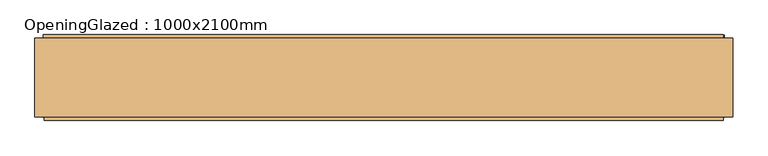
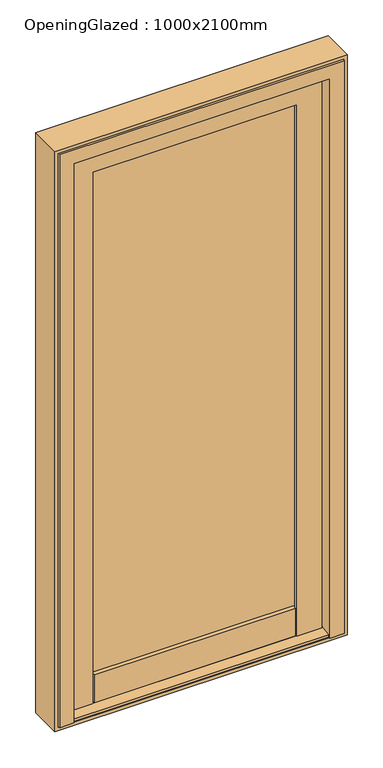
"""IFC4 building model written with IfcOpenShell, lengths in millimetres: door geometry, OpeningGlazed : 1000x2100mm."""

import ifcopenshell
import ifcopenshell.guid

model = None  # the IFC model being written
_history = None  # IfcOwnerHistory: only IFC2X3 demands one
_inside = {}  # id of a spatial element -> (the spatial element, [elements in it])
_under = {}  # id of a project, library or spatial element -> (it, [spatial elements below it])
_declared = {}  # id of a project -> (the project, [libraries it declares])
_typed = {}  # id of a type object -> (the type object, [elements of that type])
_made_of = {}  # id of a material, layer set ... -> (it, [elements and type objects made of it])


def new_model(schema):
    """Start an empty IFC model of exactly this schema.

    Asked for "IFC4X3", IfcOpenShell would pick the latest addendum, in which some entities
    have other attributes; the version numbers below select the first issue.
    IFC2X3 requires an IfcOwnerHistory on every rooted entity: one is made here for all.
    """
    global model, _history
    if schema == "IFC4X3":
        model = ifcopenshell.file(schema_version=(4, 3, 0, 0))
    else:
        model = ifcopenshell.file(schema=schema)
    _inside.clear()
    _under.clear()
    _declared.clear()
    _typed.clear()
    _made_of.clear()
    _history = None
    if model.schema == "IFC2X3":
        org = make("IfcOrganization", Name="unknown")
        user = make(
            "IfcPersonAndOrganization",
            ThePerson=make("IfcPerson", FamilyName="unknown"),
            TheOrganization=org,
        )
        app = make(
            "IfcApplication",
            ApplicationDeveloper=org,
            Version="unknown",
            ApplicationFullName="unknown",
            ApplicationIdentifier="unknown",
        )
        _history = make(
            "IfcOwnerHistory",
            OwningUser=user,
            OwningApplication=app,
            ChangeAction="ADDED",
            CreationDate=0,
        )
    return model


def make(cls, **values):
    """One entity of the class cls with the attributes given. An attribute that is None is left unset."""
    return model.create_entity(
        cls, **{name: value for name, value in values.items() if value is not None}
    )


def rooted(cls, **values):
    """An entity with a GlobalId (a new one), such as an element, a storey or a relation."""
    return make(cls, GlobalId=ifcopenshell.guid.new(), OwnerHistory=_history, **values)


def si_unit(unit_type, name, prefix=None):
    """IfcSIUnit, for example si_unit("LENGTHUNIT", "METRE", prefix="MILLI")."""
    return make("IfcSIUnit", UnitType=unit_type, Prefix=prefix, Name=name)


def assignment(units):
    """IfcUnitAssignment: the units of a project."""
    return None if units is None else make("IfcUnitAssignment", Units=units)


def point(xyz):
    """IfcCartesianPoint."""
    return None if xyz is None else make("IfcCartesianPoint", Coordinates=xyz)


def direction(xyz):
    """IfcDirection."""
    return None if xyz is None else make("IfcDirection", DirectionRatios=xyz)


def frame(location, z_axis=None, x_axis=None):
    """IfcAxis2Placement3D, a coordinate frame: its origin and axes. An axis left out is left unset."""
    return make(
        "IfcAxis2Placement3D",
        Location=point(location),
        Axis=direction(z_axis),
        RefDirection=direction(x_axis),
    )


def origin():
    """The frame at (0, 0, 0) with its axes left unset."""
    return frame((0.0, 0.0, 0.0))


def place(relative_to, where):
    """IfcLocalPlacement: puts the frame where relative to a parent placement (None: the world)."""
    return make(
        "IfcLocalPlacement", PlacementRelTo=relative_to, RelativePlacement=where
    )


def context(
    kind, dimensions, precision=None, world=None, true_north=None, identifier=None
):
    """IfcGeometricRepresentationContext, for example the 3D "Model" context."""
    return make(
        "IfcGeometricRepresentationContext",
        ContextIdentifier=identifier,
        ContextType=kind,
        CoordinateSpaceDimension=dimensions,
        Precision=precision,
        WorldCoordinateSystem=world,
        TrueNorth=true_north,
    )


def project(units=None, contexts=None):
    """IfcProject with its units and contexts."""
    return rooted(
        "IfcProject",
        Name="project",
        RepresentationContexts=contexts,
        UnitsInContext=assignment(units),
    )


def spatial(cls, under=None, at=None, **own):
    """A site, building, storey or space (cls), placed at a placement, below another one or the project."""
    s = rooted(cls, ObjectPlacement=at, **own)
    if under is not None:
        _under.setdefault(under.id(), (under, []))[1].append(s)
    return s


def polyline(points):
    """IfcPolyline through the points."""
    return make("IfcPolyline", Points=[point(p) for p in points])


def outline(outer, holes=None, kind="AREA"):
    """IfcArbitraryClosedProfileDef: a profile drawn as a closed curve; with holes, ...WithVoids."""
    if holes is None:
        return make("IfcArbitraryClosedProfileDef", ProfileType=kind, OuterCurve=outer)
    return make(
        "IfcArbitraryProfileDefWithVoids",
        ProfileType=kind,
        OuterCurve=outer,
        InnerCurves=holes,
    )


def extrude(swept, where, along, depth):
    """IfcExtrudedAreaSolid: the profile swept, set in the frame where, extruded along a direction by depth."""
    return make(
        "IfcExtrudedAreaSolid",
        SweptArea=swept,
        Position=where,
        ExtrudedDirection=direction(along),
        Depth=depth,
    )


def faces_of(points, faces, orient=None, outer=None):
    """IfcFace entities. A face is a list of loops; a loop is a list of indices into points, from 0.

    orient and outer hold one flag for each loop. By default every Orientation is true, the
    first loop of a face is its IfcFaceOuterBound and the others are IfcFaceBound.
    """
    made = []
    for i, loops in enumerate(faces):
        bounds = []
        for j, loop in enumerate(loops):
            is_outer = j == 0 if outer is None else outer[i][j]
            bounds.append(
                make(
                    "IfcFaceOuterBound" if is_outer else "IfcFaceBound",
                    Bound=make("IfcPolyLoop", Polygon=[points[k] for k in loop]),
                    Orientation=True if orient is None else orient[i][j],
                )
            )
        made.append(make("IfcFace", Bounds=bounds))
    return made


def faceted_brep(points, faces, orient=None, outer=None, voids=None):
    """IfcFacetedBrep: a solid bounded by flat faces; with voids (closed shells), ...WithVoids."""
    shared = [point(p) for p in points]
    hull = make("IfcClosedShell", CfsFaces=faces_of(shared, faces, orient, outer))
    if voids is None:
        return make("IfcFacetedBrep", Outer=hull)
    return make(
        "IfcFacetedBrepWithVoids",
        Outer=hull,
        Voids=[
            make(cls, CfsFaces=faces_of(shared, fs, o, b)) for cls, fs, o, b in voids
        ],
    )


def shape(context_of_items, identifier, shape_type, items):
    """IfcShapeRepresentation: the items that make up one representation, for example the "Body"."""
    return make(
        "IfcShapeRepresentation",
        ContextOfItems=context_of_items,
        RepresentationIdentifier=identifier,
        RepresentationType=shape_type,
        Items=items,
    )


def source(mapping_origin, context_of_items, identifier, shape_type, items):
    """IfcRepresentationMap: a shape defined once, which mapped items show again and again."""
    return make(
        "IfcRepresentationMap",
        MappingOrigin=mapping_origin,
        MappedRepresentation=shape(context_of_items, identifier, shape_type, items),
    )


def transform(
    local_origin,
    x_axis=None,
    y_axis=None,
    z_axis=None,
    scale=None,
    scale2=None,
    scale3=None,
    uniform=True,
):
    """IfcCartesianTransformationOperator3D, or its non-uniform kind. x_axis, y_axis, z_axis: its Axis1, 2, 3."""
    if uniform:
        return make(
            "IfcCartesianTransformationOperator3D",
            Axis1=direction(x_axis),
            Axis2=direction(y_axis),
            LocalOrigin=point(local_origin),
            Scale=scale,
            Axis3=direction(z_axis),
        )
    return make(
        "IfcCartesianTransformationOperator3DnonUniform",
        Axis1=direction(x_axis),
        Axis2=direction(y_axis),
        LocalOrigin=point(local_origin),
        Scale=scale,
        Axis3=direction(z_axis),
        Scale2=scale2,
        Scale3=scale3,
    )


def mapped(mapping_source, mapping_target):
    """IfcMappedItem: shows the shape of a source again, moved by a transform."""
    return make(
        "IfcMappedItem", MappingSource=mapping_source, MappingTarget=mapping_target
    )


def made_of(thing, what):
    """Note that an element or type object is made of a material, layer set ...; save() writes the relation."""
    if what is not None:
        _made_of.setdefault(what.id(), (what, []))[1].append(thing)
    return thing


def element(
    cls,
    number,
    at=None,
    inside=None,
    cuts=None,
    type_object=None,
    material=None,
    context=None,
    identifier="Body",
    shape_type=None,
    held_by="IfcProductDefinitionShape",
    body=None,
    shapes=None,
    **own,
):
    """One element of the class cls, such as IfcWall. Its Tag is "e" and its number.

    at: its placement. inside: the storey or other place that contains it. cuts: it is an
    opening in that element (IfcRelVoidsElement). A single representation is given by context,
    identifier, shape_type and body (its items); several are given by shapes. held_by: the class
    of the entity that holds the representations. save() writes the other relations.
    """
    e = rooted(cls, Tag="e%d" % number, ObjectPlacement=at, **own)
    if body is not None:
        shapes = [shape(context, identifier, shape_type, body)]
    if shapes is not None:
        e.Representation = make(held_by, Representations=shapes)
    if inside is not None:
        _inside.setdefault(inside.id(), (inside, []))[1].append(e)
    if cuts is not None:
        rooted(
            "IfcRelVoidsElement", RelatingBuildingElement=cuts, RelatedOpeningElement=e
        )
    if type_object is not None:
        _typed.setdefault(type_object.id(), (type_object, []))[1].append(e)
    return made_of(e, material)


def aggregate(whole, parts):
    """IfcRelAggregates: a whole, such as a stair, and the parts it consists of."""
    return rooted("IfcRelAggregates", RelatingObject=whole, RelatedObjects=parts)


def save(model, path):
    """Write the relations noted so far, then the file.

    IfcRelAggregates (storeys below a building ...), IfcRelContainedInSpatialStructure (elements
    in a storey), IfcRelDefinesByType, IfcRelAssociatesMaterial and IfcRelDeclares: one each for
    every whole, place, type object, material and project.
    """
    for whole, parts in _under.values():
        aggregate(whole, parts)
    for where, things in _inside.values():
        rooted(
            "IfcRelContainedInSpatialStructure",
            RelatedElements=things,
            RelatingStructure=where,
        )
    for kind, things in _typed.values():
        rooted("IfcRelDefinesByType", RelatedObjects=things, RelatingType=kind)
    for what, things in _made_of.values():
        rooted("IfcRelAssociatesMaterial", RelatedObjects=things, RelatingMaterial=what)
    for by, libraries in _declared.values():
        rooted("IfcRelDeclares", RelatingContext=by, RelatedDefinitions=libraries)
    model.write(path)


def openingglazed_1000x2100mm_71b3a25b(model_context):
    return source(origin(), model_context, "Body", "SolidModel", [
        extrude(outline(polyline([(40.9999982, 133.0208766), (48.9999995, 130.8772832), (48.9999995, 112.2614733), (47.8757378, 111.1372136), (48.9999995, 110.0129457), (48.9999995, 21.4372109), (40.9999982, 21.4372109), (40.9999982, 133.0208766)])), frame((-488.0, 0.0, 0.0), z_axis=(1.0, 0.0, 0.0), x_axis=(0.0, 1.0, 0.0)), (0.0, 0.0, 1.0), 976.0),
        extrude(outline(polyline([(-16.0, 18.5055334), (50.0, 14.6999975), (50.0, 12.0), (-65.0000006, 12.0), (-65.0000006, 21.5000005), (-28.9462261, 25.9268477), (-28.000001, 28.5265826), (-16.0, 30.0000015), (-16.0, 18.5055334)])), frame((-488.0, 0.0, 0.0), z_axis=(1.0, 0.0, 0.0), x_axis=(0.0, 1.0, 0.0)), (0.0, 0.0, 1.0), 976.0),
        extrude(outline(polyline([(40.9999982, 108.2792699), (40.9999982, 15.2189343), (-16.0, 18.5055334), (-16.0, 30.0000015), (-31.0000006, 28.1582279), (-31.0000006, 129.0), (2.9999994, 133.0), (2.9999994, 112.9450831), (40.9999982, 108.2792699)])), frame((-344.5316437, 0.0, 0.0), z_axis=(1.0, 0.0, 0.0), x_axis=(0.0, 1.0, 0.0)), (0.0, 0.0, 1.0), 689.0632873),
        extrude(outline(polyline([(358.6999971, 37.9999995), (358.6999971, 33.9999989), (-358.6999971, 33.9999989), (-358.6999971, 37.9999995), (358.6999971, 37.9999995)])), frame((0.0, 0.0, 121.9447729), z_axis=(0.0, 0.0, 1.0), x_axis=(1.0, 0.0, 0.0)), (0.0, 0.0, 1.0), 1836.7552241),
        extrude(outline(polyline([(358.6999971, -15.0000005), (358.6999971, -19.0000005), (-358.6999971, -19.0000005), (-358.6999971, -15.0000005), (358.6999971, -15.0000005)])), frame((0.0, 0.0, 121.9447729), z_axis=(0.0, 0.0, 1.0), x_axis=(1.0, 0.0, 0.0)), (0.0, 0.0, 1.0), 1836.7552241),
        extrude(outline(polyline([(2100.0, 500.0), (2100.0, -500.0), (0.0, -500.0), (0.0, 500.0), (2100.0, 500.0)]), holes=[polyline([(12.0, 488.0), (12.0, -488.0), (2088.0, -488.0), (2088.0, 488.0), (12.0, 488.0)])]), frame((0.0, -68.0, 0.0), z_axis=(0.0, 1.0, 0.0), x_axis=(0.0, 0.0, 1.0)), (0.0, 0.0, 1.0), 113.0),
        faceted_brep([(486.7916962, 41.6999992, 13.2083038), (486.7916962, -73.3, 13.2083038), (437.9999993, -73.3, 13.2083038), (437.9999993, -16.0, 13.2083038), (455.8269997, -16.0, 13.2083038), (462.9116684, 41.6999992, 13.2083038), (-486.7916962, 41.6999992, 13.2083038), (-462.9116684, 41.6999992, 13.2083038), (-455.8269997, -16.0, 13.2083038), (-437.9999993, -16.0, 13.2083038), (-437.9999993, -73.3, 13.2083038), (-486.7916962, -73.3, 13.2083038), (462.9116684, 41.6999992, 2062.9116684), (-462.9116684, 41.6999992, 2062.9116684), (-486.7916962, 41.6999992, 2086.7916962), (486.7916962, 41.6999992, 2086.7916962), (486.7916962, -73.3, 2086.7916962), (-486.7916962, -73.3, 2086.7916962), (-437.9999993, -73.3, 2037.9999993), (437.9999993, -73.3, 2037.9999993), (437.9999993, -16.0, 2037.9999993), (-437.9999993, -16.0, 2037.9999993), (-455.8269997, -16.0, 2055.8269997), (455.8269997, -16.0, 2055.8269997)], [[[0, 1, 2, 3, 4, 5]], [[6, 7, 8, 9, 10, 11]], [[0, 5, 12, 13, 7, 6, 14, 15]], [[1, 0, 15, 16]], [[2, 1, 16, 17, 11, 10, 18, 19]], [[16, 15, 14, 17]], [[17, 14, 6, 11]], [[3, 2, 19, 20]], [[4, 3, 20, 21, 9, 8, 22, 23]], [[5, 4, 23, 12]], [[20, 19, 18, 21]], [[12, 23, 22, 13]], [[21, 18, 10, 9]], [[13, 22, 8, 7]]]),
        faceted_brep([(450.532936, -11.0000001, 13.2083038), (434.0000042, -11.0000001, 13.2083038), (434.0000042, -31.0000006, 13.2083038), (348.9999993, -31.0000006, 13.2083038), (345.0, 2.9999994, 13.2083038), (365.1556953, 2.9999994, 13.2083038), (369.8215082, 40.9999982, 13.2083038), (456.9177253, 40.9999982, 13.2083038), (-450.532936, -11.0000001, 13.2083038), (-456.9177253, 40.9999982, 13.2083038), (-369.8215082, 40.9999982, 13.2083038), (-365.1556953, 2.9999994, 13.2083038), (-345.0, 2.9999994, 13.2083038), (-348.9999993, -31.0000006, 13.2083038), (-434.0000042, -31.0000006, 13.2083038), (-434.0000042, -11.0000001, 13.2083038), (450.532936, -11.0000001, 2050.532936), (-450.532936, -11.0000001, 2050.532936), (-434.0000042, -11.0000001, 2034.0000042), (434.0000042, -11.0000001, 2034.0000042), (434.0000042, -31.0000006, 2034.0000042), (-434.0000042, -31.0000006, 2034.0000042), (-348.9999993, -31.0000006, 1948.9999993), (348.9999993, -31.0000006, 1948.9999993), (345.0, 2.9999994, 1945.0), (-345.0, 2.9999994, 1945.0), (-365.1556953, 2.9999994, 1965.1556953), (365.1556953, 2.9999994, 1965.1556953), (369.8215082, 40.9999982, 1969.8215082), (-369.8215082, 40.9999982, 1969.8215082), (-456.9177253, 40.9999982, 2056.9177253), (456.9177253, 40.9999982, 2056.9177253)], [[[0, 1, 2, 3, 4, 5, 6, 7]], [[8, 9, 10, 11, 12, 13, 14, 15]], [[1, 0, 16, 17, 8, 15, 18, 19]], [[2, 1, 19, 20]], [[3, 2, 20, 21, 14, 13, 22, 23]], [[4, 3, 23, 24]], [[5, 4, 24, 25, 12, 11, 26, 27]], [[6, 5, 27, 28]], [[7, 6, 28, 29, 10, 9, 30, 31]], [[0, 7, 31, 16]], [[20, 19, 18, 21]], [[24, 23, 22, 25]], [[28, 27, 26, 29]], [[16, 31, 30, 17]], [[21, 18, 15, 14]], [[25, 22, 13, 12]], [[29, 26, 11, 10]], [[17, 30, 9, 8]]]),
        faceted_brep([(486.7916962, 41.7000007, 130.8772832), (345.267467, 41.7000007, 130.8772832), (347.2234954, 48.9999995, 130.8772832), (365.8393052, 48.9999995, 130.8772832), (366.9635649, 47.8757378, 130.8772832), (368.0878328, 48.9999995, 130.8772832), (456.6635677, 48.9999995, 130.8772832), (456.6635677, 44.5786361, 130.8772832), (463.2426434, 44.5786361, 130.8772832), (463.9083032, 50.0, 130.8772832), (486.7916962, 50.0, 130.8772832), (-488.0, 41.7000007, 130.8772832), (-488.0, 50.0, 130.8772832), (-465.116607, 50.0, 130.8772832), (-464.4509472, 44.5786361, 130.8772832), (-457.8718715, 44.5786361, 130.8772832), (-457.8718715, 48.9999995, 130.8772832), (-369.2961366, 48.9999995, 130.8772832), (-368.1718687, 47.8757378, 130.8772832), (-367.047609, 48.9999995, 130.8772832), (-348.4317991, 48.9999995, 130.8772832), (-346.4757708, 41.7000007, 130.8772832), (486.7916962, 41.7000007, 2086.7916962), (-488.0, 41.7000007, 2086.7916962), (-346.4757708, 41.7000007, 1945.267467), (345.267467, 41.7000007, 1945.267467), (347.2234954, 48.9999995, 1947.2234954), (-348.4317991, 48.9999995, 1947.2234954), (-367.047609, 48.9999995, 1965.8393052), (365.8393052, 48.9999995, 1965.8393052), (366.9635649, 47.8757378, 1966.9635649), (368.0878328, 48.9999995, 1968.0878328), (-369.2961366, 48.9999995, 1968.0878328), (-457.8718715, 48.9999995, 2056.6635677), (456.6635677, 48.9999995, 2056.6635677), (456.6635677, 44.5786361, 2056.6635677), (-457.8718715, 44.5786361, 2056.6635677), (-464.4509472, 44.5786361, 2063.2426434), (463.2426434, 44.5786361, 2063.2426434), (463.9083032, 50.0, 2063.9083032), (-465.116607, 50.0, 2063.9083032), (-488.0, 50.0, 2086.7916962), (486.7916962, 50.0, 2086.7916962), (-368.1718687, 47.8757378, 1966.9635649)], [[[0, 1, 2, 3, 4, 5, 6, 7, 8, 9, 10]], [[11, 12, 13, 14, 15, 16, 17, 18, 19, 20, 21]], [[1, 0, 22, 23, 11, 21, 24, 25]], [[2, 1, 25, 26]], [[3, 2, 26, 27, 20, 19, 28, 29]], [[4, 3, 29, 30]], [[5, 4, 30, 31]], [[6, 5, 31, 32, 17, 16, 33, 34]], [[7, 6, 34, 35]], [[8, 7, 35, 36, 15, 14, 37, 38]], [[9, 8, 38, 39]], [[10, 9, 39, 40, 13, 12, 41, 42]], [[0, 10, 42, 22]], [[26, 25, 24, 27]], [[30, 29, 28, 43]], [[31, 30, 43, 32]], [[35, 34, 33, 36]], [[39, 38, 37, 40]], [[22, 42, 41, 23]], [[27, 24, 21, 20]], [[43, 28, 19, 18]], [[32, 43, 18, 17]], [[36, 33, 16, 15]], [[40, 37, 14, 13]], [[23, 41, 12, 11]]]),
    ])


if __name__ == "__main__":
    model = new_model("IFC4")
    model_context = context("Model", 3, world=origin())
    ifc_project = project(units=[si_unit("LENGTHUNIT", "METRE", prefix="MILLI")], contexts=[model_context])
    site = spatial("IfcSite", under=ifc_project)
    building = spatial("IfcBuilding", under=site)
    placement = place(None, origin())
    openingglazed_1000x2100mm_shape = openingglazed_1000x2100mm_71b3a25b(model_context)
    element("IfcDoor", 1, ObjectType="OpeningGlazed : 1000x2100mm", at=placement, inside=building, context=model_context, shape_type="MappedRepresentation", body=[
        mapped(openingglazed_1000x2100mm_shape, transform((0.0, 0.0, 0.0), x_axis=(1.0, 0.0, 0.0), y_axis=(0.0, 1.0, 0.0), z_axis=(0.0, 0.0, 1.0))),
    ])
    save(model, "model.ifc")

# Revit data of these elements
# Type "OpeningGlazed : 1000x2100mm"
#   Type IfcGUID = "0h6TxHQWH8MRgS1iM36W8s"
#   Assembly Code = "C1020700"
#   Type Mark = "198"
#   Classification.Uniclass.EF.Number = "EF_25_30"
#   Classification.Uniclass.EF.Description = "Doors and windows"
#   WindLoadRating = "n/a"
#   WaterTightnessRating = "n/a"
#   WarrantyStartDate [instance default] = "1900-12-31T23:59:59"
#   WarrantyGuarantorParts = "n/a"
#   WarrantyGuarantorLabor = "n/a"
#   WarrantyDurationUnit = "year"
#   WarrantyDurationParts = "n/a"
#   WarrantyDurationLabor = "n/a"
#   WarrantyDescription = "n/a"
#   Version = "1"
#   Uniclass2015Version = "Products v1.9"
#   Uniclass2015Title = "Composite doorsets"
#   Uniclass2015Code = "Pr_30_59_24_16"
#   TagNumber [instance default] = "n/a"
#   SustainabilityPerformance = "n/a"
#   Status = "UNSET"
#   Size = "1000 x 2100 mm"
#   Shape = "Rectangle"
#   SerialNumber [instance default] = "n/a"
#   SecurityRating = "n/a"
#   Revision = "n/a"
#   ReplacementCost = "n/a"
#   Reference = "n/a"
#   ProductInformation = "https://velfac.co.uk/Commercial/Windows-and-doors/velfac-ribo-alu-doors/13056,2299/glazed-door-ribo-alu-edo-outward-opening"
#   Name = "CompositeDoorsets_VelfacRiboAlu-OutwardOpeningGlazed_1000x2100mm_VelfacLtd"
#   NBSReference = "45-25-28/342"
#   NBSDescription = "Composite doorsets"
#   NBSCertification = "www.nationalbimlibrary.com/cert/g5unqkvs"
#   ModelReference = "VELFAC Ribo alu - Outward opening glazed door"
#   ModelNumber = "n/a"
#   MechanicalLoadRating = "n/a"
#   Material = "Wood/ aluminium"
#   ManufacturerURL = "www.velfac.co.uk"
#   ManufacturerName = "VELFAC LTD"
#   InstallationDate [instance default] = "1900-12-31T23:59:59"
#   IfcExportType = "DOOR"
#   IfcExportAs = "IfcDoorType"
#   HygrothermalRating = "n/a"
#   Grade = "n/a"
#   GlassColor = "n/a"
#   FireRating = "n/a"
#   Finish = "n/a"
#   FillGas = "n/a"
#   Features = "n/a"
#   ExpectedLife = "n/a"
#   DurationUnit = "year"
#   DurabilityRating = "n/a"
#   DoorNumber [instance default] = "n/a"
#   Description = "Glazed entrance door in wood/ aluminium for light to medium use"
#   Contact = "Marianne Gade: mg@velfac.dk"
#   Construction Type = "ALUMINIUM_WOOD"
#   Constituents = "n/a"
#   ComponentNumber [instance default] = "n/a"
#   Comment = "U-value is based on reference window 1230 x 1480 mm. For exact U-value please contact VELFAC"
#   Color = "n/a"
#   CodePerformance = "n/a"
#   Category = "Pr_30_59_24_16:Composite doorsets"
#   BarCode [instance default] = "n/a"
#   BIMObjectName = "Vlfc_VelfacLtd_CompositeDoorsets_VelfacRiboAlu-OutwardOpeningGlazed_1000x2100mm"
#   Author = "VELFAC LTD"
#   AssetType = "Fixed"
#   AssetIdentifier [instance default] = "n/a"
#   Analytic Construction = "<None>"
#   Manufacturer = "sales-support@velfac.co.uk"
#   AcousticRating = "n/a"
#   AccessibilityPerformance = "n/a"
#   WallClosure = 0.15 m
#   VisibleLightTransmittance = 0
#   VisibleLightReflectance = 0
#   ThermalTransmittanceWinter = 0
#   ThermalTransmittanceSummer = 0
#   ThermalTransmittance = 0
#   SolarTransmittance = 0
#   SolarReflectance = 0
#   SolarHeatGainTransmittance = 0
#   SolarAbsorption = 0
#   ShadingCoefficient = 0
#   PlacementSafetyIconPlan [instance default] = 0.3 m
#   PlacementSafetyIcon = 0.827 m
#   NominalWidth = 1 m
#   NominalLength = 0 m
#   NominalHeight = 2.1 m
#   Infiltration = 0
#   GlazingBarPlacementVertical = 0.438 m
#   Uw = 0.79
#   Ug = 0.52
#   StructuralOpeningWidth = 1 m
#   StructuralOpeningHeight = 2.1 m
#   LTg = 74
#   GlazingBarPlacementHorizontalTop = 0.6 m
#   GlazingBarPlacementHorizontalMiddle = 1.05 m
#   GlazingBarPlacementHorizontalBottom = 0.6 m
#   GlazingAreaFraction = 0
#   GlassThickness3 = 0 m
#   GlassThickness2 = 0.004 m
#   GlassThickness1 = 0.004 m
#   Gg = 53
#   FrameSetback [instance default] = 0.05 m
#   Eref = 5.6
#   DoorSwingOpening [instance default] = 0.926 m
#   DoorSwing [instance default] = 90.00°
#   Rough Width = 1 m
#   Rough Height = 2.1 m
#   Joint = 0.012 m
#   Height = 2.076 m
#   Width = 0.976 m
#   SmokeStop = no
#   SelfClosing = no
#   SafetyGlassPlanSouth [instance default] = no
#   SafetyGlassPlanNorth [instance default] = no
#   SafetyGlassElevation [instance default] = no
#   IsWired = no
#   IsTempered = no
#   IsLaminated = no
#   IsExternal = yes
#   IsCoated = no
#   HasGlazingBar68mmHorizontalTop = no
#   HasGlazingBar68mmHorizontalBottom = no
#   HasDrive = no
#   HandicapAccessible = yes
#   SashOpeningRight [instance default] = yes
#   SashOpeningLeft [instance default] = yes
#   GlassLayers = 2
#   FrameDepth148mm = no
#   FrameDepth123mm = yes
#   FireExit = no
#   HasGlazingBar68mmVertical = no
#   HasGlazingBar31mmEnergyVertical = no
#   HasGlazingBar31mmEnergyHorizontalTop = no
#   HasGlazingBar31mmEnergyHorizontalBottom = no
#   HasGlazingBar68mmHorizontalMiddle = no
#   HasGlazingBar31mmEnergyHorizontalMiddle = no
#   ThresholdMaterial = Vlfc_VelfacLtd_Frame
#   GlazingPanelMaterial = Vlfc_VelfacLtd_Glass_Double
#   FrameMaterialInternal = Vlfc_VelfacLtd_Paint_White
#   FrameMaterialExternal = Vlfc_VelfacLtd_Frame
#   Type Comments = ""
#   Thickness = 0
#   Operation = ""
#   Keynote = ""
#   Fire Rating = ""
#   URL = ""
#   Model = ""
#   Function = (empty or 0)
#   Wall Closure = (empty or 0)
# Element 1 (IfcDoor, "OpeningGlazed : 1000x2100mm")
#   FrameSetback = 0 m
#   Materials on its faces: "Vlfc_VelfacLtd_Frame", "Vlfc_VelfacLtd_Paint_White", "Vlfc_VelfacLtd_Glass_Double"
# Materials
#   "Vlfc_VelfacLtd_Frame": class "Unassigned", colour RGB 80 80 80, transparency 0, Cost = 0
#   "Vlfc_VelfacLtd_Glass_Double": class "Glass", colour RGB 0 0 255, transparency 0.75, Cost = 0
#   "Vlfc_VelfacLtd_Paint_White": class "Paint/Coating", colour RGB 255 255 255, transparency 0, Cost = 0
